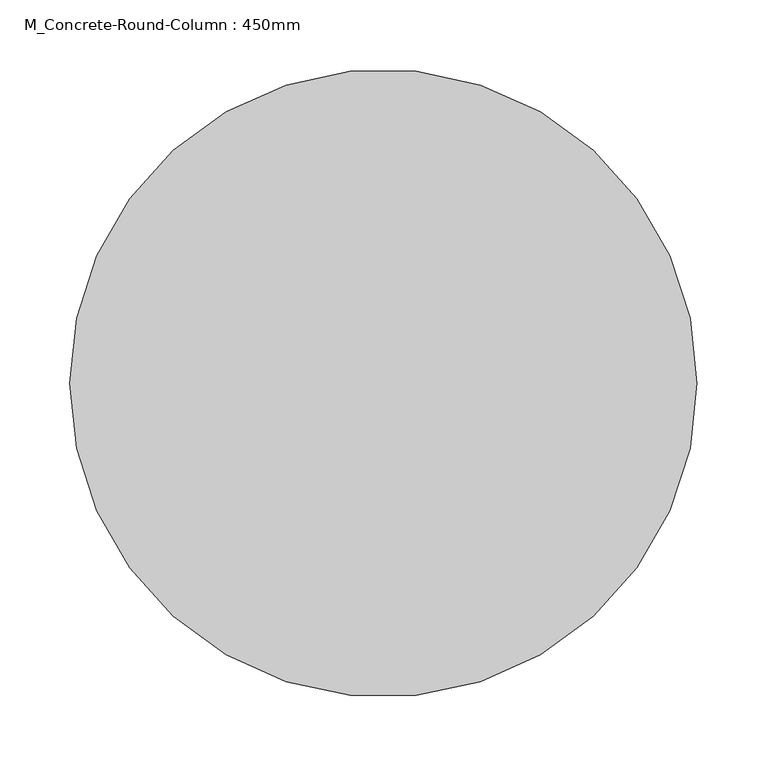
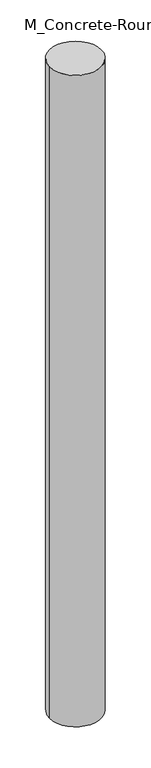
"""IFC4 building model written with IfcOpenShell, lengths in millimetres: column geometry, M_Concrete-Round-Column : 450mm."""

from ifc_helpers import new_model, si_unit, point, origin, origin_with_axes, origin_2d, place, context, project, spatial, circle_curve, trimmed, segment, composite_curve, outline, extrude, source, transform, mapped, element, save


def m_concrete_round_column_450mm_c6b5f3c9(model_context):
    return source(origin(), model_context, "Body", "SweptSolid", [
        extrude(outline(composite_curve([segment(trimmed(circle_curve(origin_2d(), 225.0), [point((-225.0, 0.0))], [point((225.0, 0.0))], False, "CARTESIAN"), True, "CONTINUOUS"), segment(trimmed(circle_curve(origin_2d(), 225.0), [point((225.0, 0.0))], [point((-225.0, 0.0))], False, "CARTESIAN"), True, "CONTINUOUS")], self_intersect=False)), origin_with_axes(), (0.0, 0.0, 1.0), 6000.0),
    ])


if __name__ == "__main__":
    model = new_model("IFC4")
    model_context = context("Model", 3, world=origin())
    ifc_project = project(units=[si_unit("LENGTHUNIT", "METRE", prefix="MILLI")], contexts=[model_context])
    site = spatial("IfcSite", under=ifc_project)
    building = spatial("IfcBuilding", under=site)
    placement = place(None, origin())
    m_concrete_round_column_450mm_shape = m_concrete_round_column_450mm_c6b5f3c9(model_context)
    element("IfcColumn", 1, ObjectType="M_Concrete-Round-Column : 450mm", at=placement, inside=building, context=model_context, shape_type="MappedRepresentation", body=[
        mapped(m_concrete_round_column_450mm_shape, transform((0.0, 0.0, 0.0), x_axis=(1.0, 0.0, 0.0), y_axis=(0.0, 1.0, 0.0), z_axis=(0.0, 0.0, 1.0))),
    ])
    save(model, "model.ifc")

# Revit data of these elements
# Type "M_Concrete-Round-Column : 450mm"
#   b = 0.45 m
#   Structural Material [instance default] = Concrete, Cast-in-Place gray
# Element 1 (IfcColumn, "M_Concrete-Round-Column : 450mm")
#   Materials on its faces: "Concrete, Cast-in-Place gray"
# Materials
#   "Concrete, Cast-in-Place gray": class "Concrete", colour RGB 192 192 192, transparency 0, Description = "Cast-in-place concrete", Cost = 0
